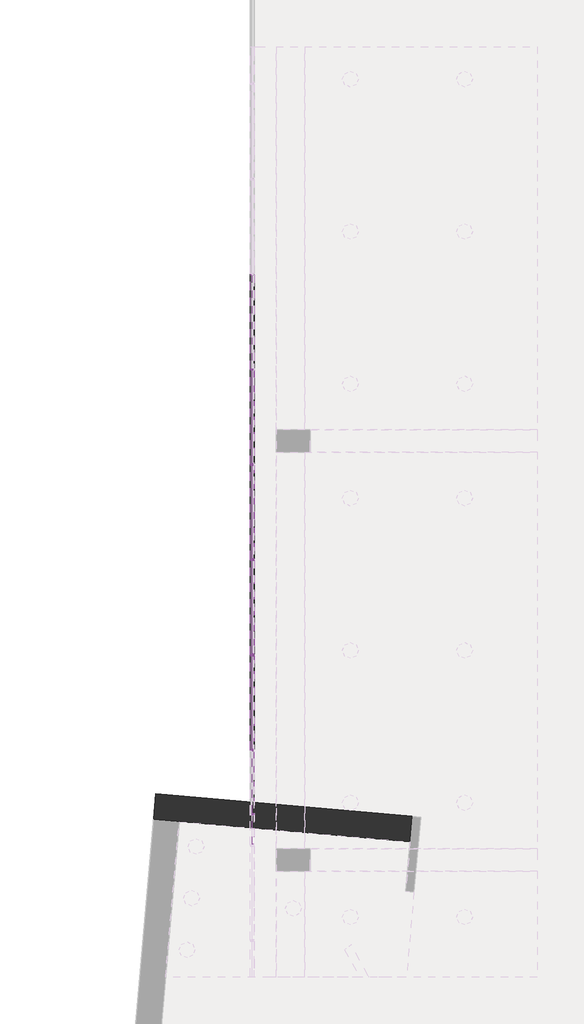
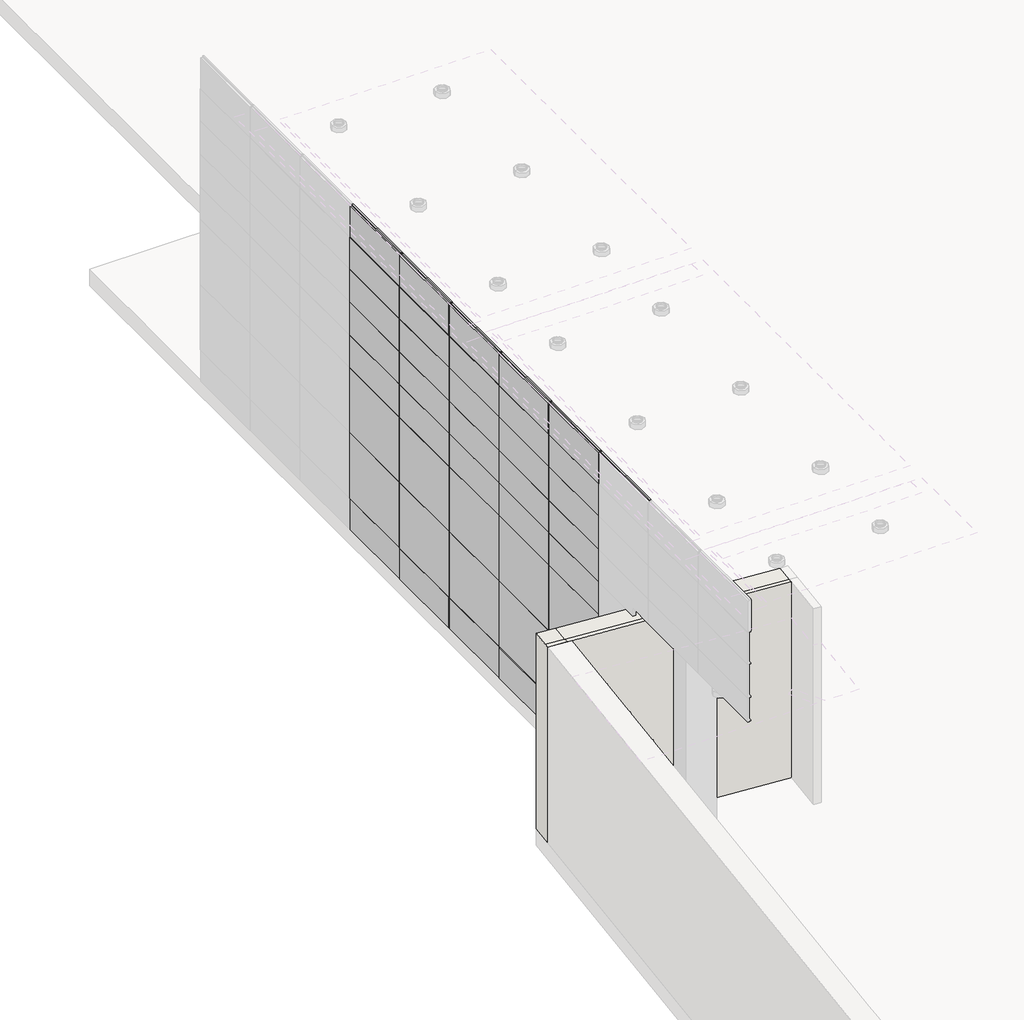
# One storey, part 6 of 30: 90 members, 40 plates, 1 wall.
# Revit data of these elements (continued)
# Project information
#   Project Issue Date = "Issue Date"
#   Project Status = "Project Status"
#   Client Name = "Owner"
#   Project Address = "Enter address here"
#   Project Name = "Project Name"
#   Project Number = "Project Number"
# Grids (mm)
#   "9.6": line (6864.976, -37283.911) -> (5806.021, -17077.846)
#   "G.5": line (37124.427, -17190.111) -> (-12577.847, -19794.897)
#   "H.5": line (37384.644, -22155.347) -> (-12317.63, -24760.133)
#   "J.5": line (37756.193, -29244.918) -> (-11946.082, -31849.704)
#   "K": line (37958.916, -33113.109) -> (-11743.358, -35717.895)
#   "F.5": line (36725.627, -9580.554) -> (10926.266, -10932.641)
#   "E.5": line (36326.827, -1970.997) -> (10527.466, -3323.084)
#   "C.5": line (35928.027, 5638.56) -> (10128.666, 4286.473)
#   "7.2": line (-9673.128, -38150.636) -> (-10732.083, -17944.571)
#   "8.4": line (-1404.076, -37717.274) -> (-2463.031, -17511.208)
#   "10.8": line (15894.983, -36810.669) -> (14836.028, -16604.603)
#   "13": line (34795.221, -35820.149) -> (33736.266, -15614.084)
#   "1": line (-51461.944, -37576.833) -> (-51461.944, 28762.958)
#   "2": line (-45365.944, -37576.833) -> (-45365.944, 28762.958)
#   "3": line (-38050.744, -37576.833) -> (-38050.744, 28762.958)
#   "4": line (-31345.144, -37576.833) -> (-31345.144, 28762.958)
#   "5": line (-24639.544, -37576.833) -> (-24639.544, 28762.958)
#   "6": line (-17933.944, -37576.833) -> (-17933.944, 28762.958)
#   "7": line (-11228.344, -37576.833) -> (-11228.344, 28762.958)
#   "8": line (-4522.744, -37576.833) -> (-4522.744, 28762.958)
#   "9": line (2182.856, -37576.833) -> (2182.856, 28762.958)
#   "10": line (8888.456, -37576.833) -> (8888.456, 28762.958)
#   "11": line (16203.656, -37576.833) -> (16203.656, 28762.958)
#   "12": line (22299.656, -37576.833) -> (22299.656, 28762.958)
#   "A": line (38014.081, 14523.24) -> (-59082, 14523.24)
#   "B": line (38014.081, 10865.64) -> (-59082, 10865.64)
#   "C": line (38014.081, 7512.84) -> (-59082, 7512.84)
#   "D": line (38014.081, 4160.04) -> (-59082, 4160.04)
#   "E": line (38014.081, 807.24) -> (-59082, 807.24)
#   "F": line (38014.081, -5898.36) -> (-59082, -5898.36)
#   "G": line (38014.081, -12603.96) -> (-59082, -12603.96)
#   "H": line (38014.081, -19309.56) -> (-59082, -19309.56)
#   "J": line (38014.081, -25405.56) -> (-59082, -25405.56)
# Type "Rectangular Mullion : 1\" Square"
#   built-in parameter 1007304 = 0.0833333 (stored number, unit not read)
#   built-in parameter 1007301 = 0.0416667 (stored number, unit not read)
#   built-in parameter 1007300 = 0.0416667 (stored number, unit not read)
# Type "Generic - 13+3 1/8\""
#   Assembly Code = "B2010"
#   Layers, outside or top first: 330.2 mm no material (function 1); 79.375 mm no material (function 1)
# Elements 1, 2, 3, 4, 5, 6, 7, 8, 9, 10, 11, 12, 13, 14, 15, 16, 17, 18, 19, 20, 21, 22, 23, 24, 25, 26, 27, 28, 29, 30, 31, 32, 33, 34, 35, 36, 37, 38, 39, 40, 41, 42, 43, 44, 45, 46, 47, 48, 49, 50, 51, 52, 53, 54, 55, 56, 57, 58, 59, 60, 61, 62, 63, 64, 65, 66, 67, 68, 69, 70, 71, 72, 73, 74, 75, 76, 77, 78, 79, 80, 81, 82, 83, 84, 85, 86, 87, 88, 89, 90 (IfcMember, "Rectangular Mullion : 1\" Square")
#   Phase Created = New Construction
#   Materials on its faces: "Metal - Aluminum"
# Elements 91, 92, 93, 94, 95, 96, 97, 98, 99, 100, 101, 102, 103, 104, 105, 106, 107, 108, 109, 110, 111, 112, 113, 114, 115, 116, 117, 118, 119, 120 (IfcPlate, "System Panel : Glazed")
#   Phase Created = New Construction
#   Materials on its faces: "Glass"
# Elements 121, 122, 123, 124, 125, 126, 127, 128, 129, 130 (IfcPlate, "System Panel : Solid")
#   Phase Created = New Construction
#   Materials on its faces: "Default"
# Element 131 (IfcWall, "Generic - 13+3 1/8\"")
#   Top Offset = 0 mm
#   Base Offset = 0 mm
#   wall height = 3657.6 mm
#   Phase Created = New Construction
#   Base Constraint = 1ST. FL.
#   Top Constraint = 2ND FL.
#   Materials on its faces: "Default Wall"
# Materials
#   "Metal - Aluminum": class "Metal", colour RGB 247 247 247, transparency 0
#   "Glass": class "Glass", colour RGB 0 128 192, transparency 0.75
#   "Default": class "Miscellaneous", colour RGB 127 127 127, transparency 0
#   "Default Wall": class "Miscellaneous", colour RGB 128 128 128, transparency 0
# Space at (-50350.74, -30466.395) mm, phase "New Construction", upper level "1ST. FL.", upper offset 3048 mm, lower offset 0 mm
#   Number = "20"
#   Name = "Space"
#   Actual Lighting Load per area = 0
#   Actual Power Load per area = 0
#   Sensible Heat Gain per person = 0
#   Specified Lighting Load = 153.554 (stored number, unit not read)
#   Specified Power Load = 199.62 (stored number, unit not read)
#   Latent Heat Gain per person = 0
#   Total Heat Gain per person = 0
#   Area per Person = 0
#   Number of People = 0.0463862 (stored number, unit not read)
#   Lighting Load Units = 0
#   Power Load Units = 0
#   Return Airflow = 0
#   Occupancy Unit = -1
#   Condition Type = 2
#   Construction Type = none
# Space at (-51280.638, -30385.039) mm, phase "New Construction", upper level "1ST. FL.", upper offset 3048 mm, lower offset 0 mm
#   Number = "21"
#   Name = "Space"
#   Actual Lighting Load per area = 0
#   Actual Power Load per area = 0
#   Sensible Heat Gain per person = 0
#   Specified Lighting Load = 153.554 (stored number, unit not read)
#   Specified Power Load = 199.62 (stored number, unit not read)
#   Latent Heat Gain per person = 0
#   Total Heat Gain per person = 0
#   Area per Person = 0
#   Number of People = 0.0463862 (stored number, unit not read)
#   Lighting Load Units = 0
#   Power Load Units = 0
#   Return Airflow = 0
#   Occupancy Unit = -1
#   Condition Type = 2
#   Construction Type = none
# Space at (-52210.536, -30303.684) mm, phase "New Construction", upper level "1ST. FL.", upper offset 3048 mm, lower offset 0 mm
#   Number = "22"
#   Name = "Space"
#   Actual Lighting Load per area = 0
#   Actual Power Load per area = 0
#   Sensible Heat Gain per person = 0
#   Specified Lighting Load = 153.554 (stored number, unit not read)
#   Specified Power Load = 199.62 (stored number, unit not read)
#   Latent Heat Gain per person = 0
#   Total Heat Gain per person = 0
#   Area per Person = 0
#   Number of People = 0.0463862 (stored number, unit not read)
#   Lighting Load Units = 0
#   Power Load Units = 0
#   Return Airflow = 0
#   Occupancy Unit = -1
#   Condition Type = 2
#   Construction Type = none
# Space at (-52088.521, -24227.572) mm, phase "New Construction", upper level "1ST. FL.", upper offset 3048 mm, lower offset 0 mm
#   Number = "23"
#   Name = "Space"
#   Actual Lighting Load per area = 0
#   Actual Power Load per area = 0
#   Sensible Heat Gain per person = 0
#   Specified Lighting Load = 3477.7 (stored number, unit not read)
#   Specified Power Load = 4521.01 (stored number, unit not read)
#   Latent Heat Gain per person = 0
#   Total Heat Gain per person = 0
#   Area per Person = 0
#   Number of People = 1.05056 (stored number, unit not read)
#   Lighting Load Units = 0
#   Power Load Units = 0
#   Return Airflow = 0
#   Occupancy Unit = -1
#   Condition Type = 2
#   Construction Type = none
# Space at (-51998.779, -31381.93) mm, phase "New Construction", upper level "1ST. FL.", upper offset 3048 mm, lower offset 0 mm
#   Number = "24"
#   Name = "Space"
#   Actual Lighting Load per area = 0
#   Actual Power Load per area = 0
#   Sensible Heat Gain per person = 0
#   Specified Lighting Load = 909.282 (stored number, unit not read)
#   Specified Power Load = 1182.07 (stored number, unit not read)
#   Latent Heat Gain per person = 0
#   Total Heat Gain per person = 0
#   Area per Person = 0
#   Number of People = 0.27468 (stored number, unit not read)
#   Lighting Load Units = 0
#   Power Load Units = 0
#   Return Airflow = 0
#   Occupancy Unit = -1
#   Condition Type = 2
#   Construction Type = none
# Space at (15225.756, -15893.26) mm, phase "New Construction", upper level "1ST. FL.", upper offset 3048 mm, lower offset 0 mm
#   Number = "29"
#   Name = "Space"
#   Actual Lighting Load per area = 0
#   Actual Power Load per area = 0
#   Sensible Heat Gain per person = 0
#   Specified Lighting Load = 62.8642 (stored number, unit not read)
#   Specified Power Load = 81.7235 (stored number, unit not read)
#   Latent Heat Gain per person = 0
#   Total Heat Gain per person = 0
#   Area per Person = 0
#   Number of People = 0.0189903 (stored number, unit not read)
#   Lighting Load Units = 0
#   Power Load Units = 0
#   Return Airflow = 0
#   Occupancy Unit = -1
#   Condition Type = 2
#   Construction Type = none
# Space at (-10682.244, -17819.949) mm, phase "New Construction", upper level "1ST. FL.", upper offset 3048 mm, lower offset 0 mm
#   Number = "30"
#   Name = "Space"
#   Actual Lighting Load per area = 0
#   Actual Power Load per area = 0
#   Sensible Heat Gain per person = 0
#   Specified Lighting Load = 1649.25 (stored number, unit not read)
#   Specified Power Load = 2144.03 (stored number, unit not read)
#   Latent Heat Gain per person = 0
#   Total Heat Gain per person = 0
#   Area per Person = 0
#   Number of People = 0.498213 (stored number, unit not read)
#   Lighting Load Units = 0
#   Power Load Units = 0
#   Return Airflow = 0
#   Occupancy Unit = -1
#   Condition Type = 2
#   Construction Type = none
# Space at (-39.644, -17389.234) mm, phase "New Construction", upper level "1ST. FL.", upper offset 3048 mm, lower offset 0 mm
#   Number = "31"
#   Name = "Space"
#   Actual Lighting Load per area = 0
#   Actual Power Load per area = 0
#   Sensible Heat Gain per person = 0
#   Specified Lighting Load = 525.995 (stored number, unit not read)
#   Specified Power Load = 683.794 (stored number, unit not read)
#   Latent Heat Gain per person = 0
#   Total Heat Gain per person = 0
#   Area per Person = 0
#   Number of People = 0.158895 (stored number, unit not read)
#   Lighting Load Units = 0
#   Power Load Units = 0
#   Return Airflow = 0
#   Occupancy Unit = -1
#   Condition Type = 2
#   Construction Type = none
# Space at (2182.856, 13850.14) mm, phase "New Construction", upper level "1ST. FL.", upper offset 3048 mm, lower offset 0 mm
#   Number = "36"
#   Name = "Space"
#   Actual Lighting Load per area = 0
#   Actual Power Load per area = 0
#   Sensible Heat Gain per person = 0
#   Specified Lighting Load = 134.399 (stored number, unit not read)
#   Specified Power Load = 174.719 (stored number, unit not read)
#   Latent Heat Gain per person = 0
#   Total Heat Gain per person = 0
#   Area per Person = 0
#   Number of People = 0.0405999 (stored number, unit not read)
#   Lighting Load Units = 0
#   Power Load Units = 0
#   Return Airflow = 0
#   Occupancy Unit = -1
#   Condition Type = 2
#   Construction Type = none
# Space at (-44388.044, -15893.26) mm, phase "New Construction", upper level "1ST. FL.", upper offset 3048 mm, lower offset 0 mm
#   Number = "37"
#   Name = "Space"
#   Actual Lighting Load per area = 0
#   Actual Power Load per area = 0
#   Sensible Heat Gain per person = 0
#   Specified Lighting Load = 62.8642 (stored number, unit not read)
#   Specified Power Load = 81.7235 (stored number, unit not read)
#   Latent Heat Gain per person = 0
#   Total Heat Gain per person = 0
#   Area per Person = 0
#   Number of People = 0.0189903 (stored number, unit not read)
#   Lighting Load Units = 0
#   Power Load Units = 0
#   Return Airflow = 0
#   Occupancy Unit = -1
#   Condition Type = 2
#   Construction Type = none
# Space at (-31345.144, 13850.14) mm, phase "New Construction", upper level "1ST. FL.", upper offset 3048 mm, lower offset 0 mm
#   Number = "40"
#   Name = "Space"
#   Actual Lighting Load per area = 0
#   Actual Power Load per area = 0
#   Sensible Heat Gain per person = 0
#   Specified Lighting Load = 134.399 (stored number, unit not read)
#   Specified Power Load = 174.719 (stored number, unit not read)
#   Latent Heat Gain per person = 0
#   Total Heat Gain per person = 0
#   Area per Person = 0
#   Number of People = 0.0405999 (stored number, unit not read)
#   Lighting Load Units = 0
#   Power Load Units = 0
#   Return Airflow = 0
#   Occupancy Unit = -1
#   Condition Type = 2
#   Construction Type = none
# Space at (-14581.144, -2215.36) mm, phase "New Construction", upper level "1ST. FL.", upper offset 3048 mm, lower offset 0 mm
#   Number = "41"
#   Name = "Space"
#   Actual Lighting Load per area = 0
#   Actual Power Load per area = 0
#   Sensible Heat Gain per person = 0
#   Specified Lighting Load = 213384.3 (stored number, unit not read)
#   Specified Power Load = 277399.6 (stored number, unit not read)
#   Latent Heat Gain per person = 0
#   Total Heat Gain per person = 0
#   Area per Person = 0
#   Number of People = 64.46 (stored number, unit not read)
#   Lighting Load Units = 0
#   Power Load Units = 0
#   Return Airflow = 0
#   Occupancy Unit = -1
#   Condition Type = 2
#   Construction Type = none
# Space at (-22969.494, 18968.24) mm, phase "New Construction", upper level "1ST. FL.", upper offset 3048 mm, lower offset 0 mm
#   Number = "44"
#   Name = "Space"
#   Actual Lighting Load per area = 0
#   Actual Power Load per area = 0
#   Sensible Heat Gain per person = 0
#   Specified Lighting Load = 1066.26 (stored number, unit not read)
#   Specified Power Load = 1386.14 (stored number, unit not read)
#   Latent Heat Gain per person = 0
#   Total Heat Gain per person = 0
#   Area per Person = 0
#   Number of People = 0.322101 (stored number, unit not read)
#   Lighting Load Units = 0
#   Power Load Units = 0
#   Return Airflow = 0
#   Occupancy Unit = -1
#   Condition Type = 2
#   Construction Type = none
# Space at (-19896.094, 18968.24) mm, phase "New Construction", upper level "1ST. FL.", upper offset 3048 mm, lower offset 0 mm
#   Number = "45"
#   Name = "Space"
#   Actual Lighting Load per area = 0
#   Actual Power Load per area = 0
#   Sensible Heat Gain per person = 0
#   Specified Lighting Load = 560.359 (stored number, unit not read)
#   Specified Power Load = 728.466 (stored number, unit not read)
#   Latent Heat Gain per person = 0
#   Total Heat Gain per person = 0
#   Area per Person = 0
#   Number of People = 0.169275 (stored number, unit not read)
#   Lighting Load Units = 0
#   Power Load Units = 0
#   Return Airflow = 0
#   Occupancy Unit = -1
#   Condition Type = 2
#   Construction Type = none
# Space at (-18559.419, 18968.24) mm, phase "New Construction", upper level "1ST. FL.", upper offset 3048 mm, lower offset 0 mm
#   Number = "46"
#   Name = "Space"
#   Actual Lighting Load per area = 0
#   Actual Power Load per area = 0
#   Sensible Heat Gain per person = 0
#   Specified Lighting Load = 99.2485 (stored number, unit not read)
#   Specified Power Load = 129.023 (stored number, unit not read)
#   Latent Heat Gain per person = 0
#   Total Heat Gain per person = 0
#   Area per Person = 0
#   Number of People = 0.0299814 (stored number, unit not read)
#   Lighting Load Units = 0
#   Power Load Units = 0
#   Return Airflow = 0
#   Occupancy Unit = -1
#   Condition Type = 2
#   Construction Type = none
# Space at (-33885.144, 21730.49) mm, phase "New Construction", upper level "1ST. FL.", upper offset 3048 mm, lower offset 0 mm
#   Number = "47"
#   Name = "Space"
#   Actual Lighting Load per area = 0
#   Actual Power Load per area = 0
#   Sensible Heat Gain per person = 0
#   Specified Lighting Load = 18748.3 (stored number, unit not read)
#   Specified Power Load = 24372.8 (stored number, unit not read)
#   Latent Heat Gain per person = 0
#   Total Heat Gain per person = 0
#   Area per Person = 0
#   Number of People = 5.66358 (stored number, unit not read)
#   Lighting Load Units = 0
#   Power Load Units = 0
#   Return Airflow = 0
#   Occupancy Unit = -1
#   Condition Type = 2
#   Construction Type = none
# Space at (-34520.144, 24245.09) mm, phase "New Construction", upper level "1ST. FL.", upper offset 3048 mm, lower offset 0 mm
#   Number = "48"
#   Name = "Space"
#   Actual Lighting Load per area = 0
#   Actual Power Load per area = 0
#   Sensible Heat Gain per person = 0
#   Specified Lighting Load = 746.746 (stored number, unit not read)
#   Specified Power Load = 970.77 (stored number, unit not read)
#   Latent Heat Gain per person = 0
#   Total Heat Gain per person = 0
#   Area per Person = 0
#   Number of People = 0.22558 (stored number, unit not read)
#   Lighting Load Units = 0
#   Power Load Units = 0
#   Return Airflow = 0
#   Occupancy Unit = -1
#   Condition Type = 2
#   Construction Type = none
# Space at (-32361.144, 24245.09) mm, phase "New Construction", upper level "1ST. FL.", upper offset 3048 mm, lower offset 0 mm
#   Number = "49"
#   Name = "Space"
#   Actual Lighting Load per area = 0
#   Actual Power Load per area = 0
#   Sensible Heat Gain per person = 0
#   Specified Lighting Load = 547.614 (stored number, unit not read)
#   Specified Power Load = 711.898 (stored number, unit not read)
#   Latent Heat Gain per person = 0
#   Total Heat Gain per person = 0
#   Area per Person = 0
#   Number of People = 0.165425 (stored number, unit not read)
#   Lighting Load Units = 0
#   Power Load Units = 0
#   Return Airflow = 0
#   Occupancy Unit = -1
#   Condition Type = 2
#   Construction Type = none
# Space at (-29490.944, 24245.09) mm, phase "New Construction", upper level "1ST. FL.", upper offset 3048 mm, lower offset 0 mm
#   Number = "50"
#   Name = "Space"
#   Actual Lighting Load per area = 0
#   Actual Power Load per area = 0
#   Sensible Heat Gain per person = 0
#   Specified Lighting Load = 1211.39 (stored number, unit not read)
#   Specified Power Load = 1574.8 (stored number, unit not read)
#   Latent Heat Gain per person = 0
#   Total Heat Gain per person = 0
#   Area per Person = 0
#   Number of People = 0.365941 (stored number, unit not read)
#   Lighting Load Units = 0
#   Power Load Units = 0
#   Return Airflow = 0
#   Occupancy Unit = -1
#   Condition Type = 2
#   Construction Type = none
# Space at (-20670.794, 24245.09) mm, phase "New Construction", upper level "1ST. FL.", upper offset 3048 mm, lower offset 0 mm
#   Number = "51"
#   Name = "Space"
#   Actual Lighting Load per area = 0
#   Actual Power Load per area = 0
#   Sensible Heat Gain per person = 0
#   Specified Lighting Load = 1510.09 (stored number, unit not read)
#   Specified Power Load = 1963.11 (stored number, unit not read)
#   Latent Heat Gain per person = 0
#   Total Heat Gain per person = 0
#   Area per Person = 0
#   Number of People = 0.456173 (stored number, unit not read)
#   Lighting Load Units = 0
#   Power Load Units = 0
#   Return Airflow = 0
#   Occupancy Unit = -1
#   Condition Type = 2
#   Construction Type = none
# Space at (15876.631, 9189.24) mm, phase "New Construction", upper level "1ST. FL.", upper offset 3048 mm, lower offset 0 mm
#   Number = "53"
#   Name = "Space"
#   Actual Lighting Load per area = 0
#   Actual Power Load per area = 0
#   Sensible Heat Gain per person = 0
#   Specified Lighting Load = 68.1434 (stored number, unit not read)
#   Specified Power Load = 88.5864 (stored number, unit not read)
#   Latent Heat Gain per person = 0
#   Total Heat Gain per person = 0
#   Area per Person = 0
#   Number of People = 0.020585 (stored number, unit not read)
#   Lighting Load Units = 0
#   Power Load Units = 0
#   Return Airflow = 0
#   Occupancy Unit = -1
#   Condition Type = 2
#   Construction Type = none
# Space at (15876.631, 6550.815) mm, phase "New Construction", upper level "1ST. FL.", upper offset 3048 mm, lower offset 0 mm
#   Number = "54"
#   Name = "Space"
#   Actual Lighting Load per area = 0
#   Actual Power Load per area = 0
#   Sensible Heat Gain per person = 0
#   Specified Lighting Load = 33.455 (stored number, unit not read)
#   Specified Power Load = 43.4915 (stored number, unit not read)
#   Latent Heat Gain per person = 0
#   Total Heat Gain per person = 0
#   Area per Person = 0
#   Number of People = 0.0101062 (stored number, unit not read)
#   Lighting Load Units = 0
#   Power Load Units = 0
#   Return Airflow = 0
#   Occupancy Unit = -1
#   Condition Type = 2
#   Construction Type = none
# Space at (-5629.232, 19134.928) mm, phase "New Construction", upper level "1ST. FL.", upper offset 3048 mm, lower offset 0 mm
#   Number = "55"
#   Name = "Space"
#   Actual Lighting Load per area = 0
#   Actual Power Load per area = 0
#   Sensible Heat Gain per person = 0
#   Specified Lighting Load = 837.567 (stored number, unit not read)
#   Specified Power Load = 1088.84 (stored number, unit not read)
#   Latent Heat Gain per person = 0
#   Total Heat Gain per person = 0
#   Area per Person = 0
#   Number of People = 0.253016 (stored number, unit not read)
#   Lighting Load Units = 0
#   Power Load Units = 0
#   Return Airflow = 0
#   Occupancy Unit = -1
#   Condition Type = 2
#   Construction Type = none
# Space at (5749.822, 21730.49) mm, phase "New Construction", upper level "1ST. FL.", upper offset 3048 mm, lower offset 0 mm
#   Number = "56"
#   Name = "Space"
#   Actual Lighting Load per area = 0
#   Actual Power Load per area = 0
#   Sensible Heat Gain per person = 0
#   Specified Lighting Load = 21109.8 (stored number, unit not read)
#   Specified Power Load = 27442.8 (stored number, unit not read)
#   Latent Heat Gain per person = 0
#   Total Heat Gain per person = 0
#   Area per Person = 0
#   Number of People = 6.37694 (stored number, unit not read)
#   Lighting Load Units = 0
#   Power Load Units = 0
#   Return Airflow = 0
#   Occupancy Unit = -1
#   Condition Type = 2
#   Construction Type = none
# Space at (-8974.094, 22176.578) mm, phase "New Construction", upper level "1ST. FL.", upper offset 3048 mm, lower offset 0 mm
#   Number = "57"
#   Name = "Space"
#   Actual Lighting Load per area = 0
#   Actual Power Load per area = 0
#   Sensible Heat Gain per person = 0
#   Specified Lighting Load = 2957.38 (stored number, unit not read)
#   Specified Power Load = 3844.6 (stored number, unit not read)
#   Latent Heat Gain per person = 0
#   Total Heat Gain per person = 0
#   Area per Person = 0
#   Number of People = 0.893379 (stored number, unit not read)
#   Lighting Load Units = 0
#   Power Load Units = 0
#   Return Airflow = 0
#   Occupancy Unit = -1
#   Condition Type = 2
#   Construction Type = none
# Space at (-44969.069, -12603.96) mm, phase "New Construction", upper level "1ST. FL.", upper offset 3048 mm, lower offset 0 mm
#   Number = "58"
#   Name = "Space"
#   Actual Lighting Load per area = 0
#   Actual Power Load per area = 0
#   Sensible Heat Gain per person = 0
#   Specified Lighting Load = 3.50388 (stored number, unit not read)
#   Specified Power Load = 4.55504 (stored number, unit not read)
#   Latent Heat Gain per person = 0
#   Total Heat Gain per person = 0
#   Area per Person = 0
#   Number of People = 0.00105847 (stored number, unit not read)
#   Lighting Load Units = 0
#   Power Load Units = 0
#   Return Airflow = 0
#   Occupancy Unit = -1
#   Condition Type = 2
#   Construction Type = none
# Space at (-42459.607, -28070.561) mm, phase "New Construction", upper level "1ST. FL.", upper offset 3048 mm, lower offset 0 mm
#   Number = "59"
#   Name = "Space"
#   Actual Lighting Load per area = 0
#   Actual Power Load per area = 0
#   Sensible Heat Gain per person = 0
#   Specified Lighting Load = 2731.52 (stored number, unit not read)
#   Specified Power Load = 3550.97 (stored number, unit not read)
#   Latent Heat Gain per person = 0
#   Total Heat Gain per person = 0
#   Area per Person = 0
#   Number of People = 0.825148 (stored number, unit not read)
#   Lighting Load Units = 0
#   Power Load Units = 0
#   Return Airflow = 0
#   Occupancy Unit = -1
#   Condition Type = 2
#   Construction Type = none
# Space at (15806.781, 807.24) mm, phase "New Construction", upper level "1ST. FL.", upper offset 3048 mm, lower offset 0 mm
#   Number = "62"
#   Name = "Space"
#   Actual Lighting Load per area = 0
#   Actual Power Load per area = 0
#   Sensible Heat Gain per person = 0
#   Specified Lighting Load = 3.50388 (stored number, unit not read)
#   Specified Power Load = 4.55504 (stored number, unit not read)
#   Latent Heat Gain per person = 0
#   Total Heat Gain per person = 0
#   Area per Person = 0
#   Number of People = 0.00105847 (stored number, unit not read)
#   Lighting Load Units = 0
#   Power Load Units = 0
#   Return Airflow = 0
#   Occupancy Unit = -1
#   Condition Type = 2
#   Construction Type = none
# Space at (-44969.069, -5898.36) mm, phase "New Construction", upper level "1ST. FL.", upper offset 3048 mm, lower offset 0 mm
#   Number = "63"
#   Name = "Space"
#   Actual Lighting Load per area = 0
#   Actual Power Load per area = 0
#   Sensible Heat Gain per person = 0
#   Specified Lighting Load = 3.50388 (stored number, unit not read)
#   Specified Power Load = 4.55504 (stored number, unit not read)
#   Latent Heat Gain per person = 0
#   Total Heat Gain per person = 0
#   Area per Person = 0
#   Number of People = 0.00105847 (stored number, unit not read)
#   Lighting Load Units = 0
#   Power Load Units = 0
#   Return Airflow = 0
#   Occupancy Unit = -1
#   Condition Type = 2
#   Construction Type = none
# Space at (-44969.069, 807.24) mm, phase "New Construction", upper level "1ST. FL.", upper offset 3048 mm, lower offset 0 mm
#   Number = "64"
#   Name = "Space"
#   Actual Lighting Load per area = 0
#   Actual Power Load per area = 0
#   Sensible Heat Gain per person = 0
#   Specified Lighting Load = 3.50388 (stored number, unit not read)
#   Specified Power Load = 4.55504 (stored number, unit not read)
#   Latent Heat Gain per person = 0
#   Total Heat Gain per person = 0
#   Area per Person = 0
#   Number of People = 0.00105847 (stored number, unit not read)
#   Lighting Load Units = 0
#   Power Load Units = 0
#   Return Airflow = 0
#   Occupancy Unit = -1
#   Condition Type = 2
#   Construction Type = none
# Space at (-15300.665, 15209.103) mm, phase "New Construction", upper level "1ST. FL.", upper offset 3048 mm, lower offset 0 mm
#   Number = "65"
#   Name = "Space"
#   Actual Lighting Load per area = 0
#   Actual Power Load per area = 0
#   Sensible Heat Gain per person = 0
#   Specified Lighting Load = 29471.5 (stored number, unit not read)
#   Specified Power Load = 38312.9 (stored number, unit not read)
#   Latent Heat Gain per person = 0
#   Total Heat Gain per person = 0
#   Area per Person = 0
#   Number of People = 8.90286 (stored number, unit not read)
#   Lighting Load Units = 0
#   Power Load Units = 0
#   Return Airflow = 0
#   Occupancy Unit = -1
#   Condition Type = 2
#   Construction Type = none
# Space at (15806.781, 10865.64) mm, phase "New Construction", upper level "1ST. FL.", upper offset 3048 mm, lower offset 0 mm
#   Number = "66"
#   Name = "Space"
#   Actual Lighting Load per area = 0
#   Actual Power Load per area = 0
#   Sensible Heat Gain per person = 0
#   Specified Lighting Load = 3.50388 (stored number, unit not read)
#   Specified Power Load = 4.55504 (stored number, unit not read)
#   Latent Heat Gain per person = 0
#   Total Heat Gain per person = 0
#   Area per Person = 0
#   Number of People = 0.00105847 (stored number, unit not read)
#   Lighting Load Units = 0
#   Power Load Units = 0
#   Return Airflow = 0
#   Occupancy Unit = -1
#   Condition Type = 2
#   Construction Type = none
# Space at (15806.781, 7512.84) mm, phase "New Construction", upper level "1ST. FL.", upper offset 3048 mm, lower offset 0 mm
#   Number = "67"
#   Name = "Space"
#   Actual Lighting Load per area = 0
#   Actual Power Load per area = 0
#   Sensible Heat Gain per person = 0
#   Specified Lighting Load = 3.50388 (stored number, unit not read)
#   Specified Power Load = 4.55504 (stored number, unit not read)
#   Latent Heat Gain per person = 0
#   Total Heat Gain per person = 0
#   Area per Person = 0
#   Number of People = 0.00105847 (stored number, unit not read)
#   Lighting Load Units = 0
#   Power Load Units = 0
#   Return Airflow = 0
#   Occupancy Unit = -1
#   Condition Type = 2
#   Construction Type = none
# Space at (-44969.069, 7512.84) mm, phase "New Construction", upper level "1ST. FL.", upper offset 3048 mm, lower offset 0 mm
#   Number = "68"
#   Name = "Space"
#   Actual Lighting Load per area = 0
#   Actual Power Load per area = 0
#   Sensible Heat Gain per person = 0
#   Specified Lighting Load = 3.50388 (stored number, unit not read)
#   Specified Power Load = 4.55504 (stored number, unit not read)
#   Latent Heat Gain per person = 0
#   Total Heat Gain per person = 0
#   Area per Person = 0
#   Number of People = 0.00105847 (stored number, unit not read)
#   Lighting Load Units = 0
#   Power Load Units = 0
#   Return Airflow = 0
#   Occupancy Unit = -1
#   Condition Type = 2
#   Construction Type = none
# Space at (-44969.069, 4160.04) mm, phase "New Construction", upper level "1ST. FL.", upper offset 3048 mm, lower offset 0 mm
#   Number = "69"
#   Name = "Space"
#   Actual Lighting Load per area = 0
#   Actual Power Load per area = 0
#   Sensible Heat Gain per person = 0
#   Specified Lighting Load = 3.50388 (stored number, unit not read)
#   Specified Power Load = 4.55504 (stored number, unit not read)
#   Latent Heat Gain per person = 0
#   Total Heat Gain per person = 0
#   Area per Person = 0
#   Number of People = 0.00105847 (stored number, unit not read)
#   Lighting Load Units = 0
#   Power Load Units = 0
#   Return Airflow = 0
#   Occupancy Unit = -1
#   Condition Type = 2
#   Construction Type = none
# Space at (-2305.302, -27806.676) mm, phase "New Construction", upper level "1ST. FL.", upper offset 3048 mm, lower offset 0 mm
#   Number = "70"
#   Name = "Space"
#   Actual Lighting Load per area = 0
#   Actual Power Load per area = 0
#   Sensible Heat Gain per person = 0
#   Specified Lighting Load = 979.316 (stored number, unit not read)
#   Specified Power Load = 1273.11 (stored number, unit not read)
#   Latent Heat Gain per person = 0
#   Total Heat Gain per person = 0
#   Area per Person = 0
#   Number of People = 0.295836 (stored number, unit not read)
#   Lighting Load Units = 0
#   Power Load Units = 0
#   Return Airflow = 0
#   Occupancy Unit = -1
#   Condition Type = 2
#   Construction Type = none
# Space at (427.548, -27351.224) mm, phase "New Construction", upper level "1ST. FL.", upper offset 3048 mm, lower offset 0 mm
#   Number = "71"
#   Name = "Space"
#   Actual Lighting Load per area = 0
#   Actual Power Load per area = 0
#   Sensible Heat Gain per person = 0
#   Specified Lighting Load = 1259.38 (stored number, unit not read)
#   Specified Power Load = 1637.19 (stored number, unit not read)
#   Latent Heat Gain per person = 0
#   Total Heat Gain per person = 0
#   Area per Person = 0
#   Number of People = 0.380438 (stored number, unit not read)
#   Lighting Load Units = 0
#   Power Load Units = 0
#   Return Airflow = 0
#   Occupancy Unit = -1
#   Condition Type = 2
#   Construction Type = none
# Space at (287.151, -24805.774) mm, phase "New Construction", upper level "1ST. FL.", upper offset 3048 mm, lower offset 0 mm
#   Number = "72"
#   Name = "Space"
#   Actual Lighting Load per area = 0
#   Actual Power Load per area = 0
#   Sensible Heat Gain per person = 0
#   Specified Lighting Load = 285.033 (stored number, unit not read)
#   Specified Power Load = 370.542 (stored number, unit not read)
#   Latent Heat Gain per person = 0
#   Total Heat Gain per person = 0
#   Area per Person = 0
#   Number of People = 0.0861038 (stored number, unit not read)
#   Lighting Load Units = 0
#   Power Load Units = 0
#   Return Airflow = 0
#   Occupancy Unit = -1
#   Condition Type = 2
#   Construction Type = none
# Space at (-4916.12, -27061.973) mm, phase "New Construction", upper level "1ST. FL.", upper offset 3048 mm, lower offset 0 mm
#   Number = "73"
#   Name = "Space"
#   Actual Lighting Load per area = 0
#   Actual Power Load per area = 0
#   Sensible Heat Gain per person = 0
#   Specified Lighting Load = 1376.65 (stored number, unit not read)
#   Specified Power Load = 1789.64 (stored number, unit not read)
#   Latent Heat Gain per person = 0
#   Total Heat Gain per person = 0
#   Area per Person = 0
#   Number of People = 0.415864 (stored number, unit not read)
#   Lighting Load Units = 0
#   Power Load Units = 0
#   Return Airflow = 0
#   Occupancy Unit = -1
#   Condition Type = 2
#   Construction Type = none
# Space at (-6193.624, -24385.796) mm, phase "New Construction", upper level "1ST. FL.", upper offset 3048 mm, lower offset 0 mm
#   Number = "74"
#   Name = "Space"
#   Actual Lighting Load per area = 0
#   Actual Power Load per area = 0
#   Sensible Heat Gain per person = 0
#   Specified Lighting Load = 3.99747 (stored number, unit not read)
#   Specified Power Load = 5.19671 (stored number, unit not read)
#   Latent Heat Gain per person = 0
#   Total Heat Gain per person = 0
#   Area per Person = 0
#   Number of People = 0.00120757 (stored number, unit not read)
#   Lighting Load Units = 0
#   Power Load Units = 0
#   Return Airflow = 0
#   Occupancy Unit = -1
#   Condition Type = 2
#   Construction Type = none
# Space at (-4171.546, -33504.071) mm, phase "New Construction", upper level "1ST. FL.", upper offset 3048 mm, lower offset 0 mm
#   Number = "75"
#   Name = "Space"
#   Actual Lighting Load per area = 0
#   Actual Power Load per area = 0
#   Sensible Heat Gain per person = 0
#   Specified Lighting Load = 1778.74 (stored number, unit not read)
#   Specified Power Load = 2312.36 (stored number, unit not read)
#   Latent Heat Gain per person = 0
#   Total Heat Gain per person = 0
#   Area per Person = 0
#   Number of People = 0.537328 (stored number, unit not read)
#   Lighting Load Units = 0
#   Power Load Units = 0
#   Return Airflow = 0
#   Occupancy Unit = -1
#   Condition Type = 2
#   Construction Type = none
# Space at (3097.933, -26775.812) mm, phase "New Construction", upper level "1ST. FL.", upper offset 3048 mm, lower offset 0 mm
#   Number = "76"
#   Name = "Space"
#   Actual Lighting Load per area = 0
#   Actual Power Load per area = 0
#   Sensible Heat Gain per person = 0
#   Specified Lighting Load = 1438.51 (stored number, unit not read)
#   Specified Power Load = 1870.07 (stored number, unit not read)
#   Latent Heat Gain per person = 0
#   Total Heat Gain per person = 0
#   Area per Person = 0
#   Number of People = 0.434552 (stored number, unit not read)
#   Lighting Load Units = 0
#   Power Load Units = 0
#   Return Airflow = 0
#   Occupancy Unit = -1
#   Condition Type = 2
#   Construction Type = none
# Space at (15459.645, -28932.095) mm, phase "New Construction", upper level "1ST. FL.", upper offset 3048 mm, lower offset 0 mm
#   Number = "77"
#   Name = "Space"
#   Actual Lighting Load per area = 0
#   Actual Power Load per area = 0
#   Sensible Heat Gain per person = 0
#   Specified Lighting Load = 102.724 (stored number, unit not read)
#   Specified Power Load = 133.541 (stored number, unit not read)
#   Latent Heat Gain per person = 0
#   Total Heat Gain per person = 0
#   Area per Person = 0
#   Number of People = 0.0310313 (stored number, unit not read)
#   Lighting Load Units = 0
#   Power Load Units = 0
#   Return Airflow = 0
#   Occupancy Unit = -1
#   Condition Type = 2
#   Construction Type = none
# Space at (14240.113, -29014.839) mm, phase "New Construction", upper level "1ST. FL.", upper offset 3048 mm, lower offset 0 mm
#   Number = "78"
#   Name = "Space"
#   Actual Lighting Load per area = 0
#   Actual Power Load per area = 0
#   Sensible Heat Gain per person = 0
#   Specified Lighting Load = 533.711 (stored number, unit not read)
#   Specified Power Load = 693.824 (stored number, unit not read)
#   Latent Heat Gain per person = 0
#   Total Heat Gain per person = 0
#   Area per Person = 0
#   Number of People = 0.161225 (stored number, unit not read)
#   Lighting Load Units = 0
#   Power Load Units = 0
#   Return Airflow = 0
#   Occupancy Unit = -1
#   Condition Type = 2
#   Construction Type = none
# Space at (12037.866, -27791.919) mm, phase "New Construction", upper level "1ST. FL.", upper offset 3048 mm, lower offset 0 mm
#   Number = "79"
#   Name = "Space"
#   Actual Lighting Load per area = 0
#   Actual Power Load per area = 0
#   Sensible Heat Gain per person = 0
#   Specified Lighting Load = 40.5614 (stored number, unit not read)
#   Specified Power Load = 52.7299 (stored number, unit not read)
#   Latent Heat Gain per person = 0
#   Total Heat Gain per person = 0
#   Area per Person = 0
#   Number of People = 0.012253 (stored number, unit not read)
#   Lighting Load Units = 0
#   Power Load Units = 0
#   Return Airflow = 0
#   Occupancy Unit = -1
#   Condition Type = 2
#   Construction Type = none
# Space at (1956.988, -29737.289) mm, phase "New Construction", upper level "1ST. FL.", upper offset 3048 mm, lower offset 0 mm
#   Number = "80"
#   Name = "Space"
#   Actual Lighting Load per area = 0
#   Actual Power Load per area = 0
#   Sensible Heat Gain per person = 0
#   Specified Lighting Load = 9441.92 (stored number, unit not read)
#   Specified Power Load = 12274.5 (stored number, unit not read)
#   Latent Heat Gain per person = 0
#   Total Heat Gain per person = 0
#   Area per Person = 0
#   Number of People = 2.85225 (stored number, unit not read)
#   Lighting Load Units = 0
#   Power Load Units = 0
#   Return Airflow = 0
#   Occupancy Unit = -1
#   Condition Type = 2
#   Construction Type = none
# Space at (21735.466, 4888.703) mm, phase "New Construction", upper level "1ST. FL.", upper offset 3048 mm, lower offset 0 mm
#   Number = "81"
#   Name = "Space"
#   Actual Lighting Load per area = 0
#   Actual Power Load per area = 0
#   Sensible Heat Gain per person = 0
#   Specified Lighting Load = 193.227 (stored number, unit not read)
#   Specified Power Load = 251.196 (stored number, unit not read)
#   Latent Heat Gain per person = 0
#   Total Heat Gain per person = 0
#   Area per Person = 0
#   Number of People = 0.0583709 (stored number, unit not read)
#   Lighting Load Units = 0
#   Power Load Units = 0
#   Return Airflow = 0
#   Occupancy Unit = -1
#   Condition Type = 2
#   Construction Type = none
# Space at (22320.008, -16889.371) mm, phase "New Construction", upper level "1ST. FL.", upper offset 3048 mm, lower offset 0 mm
#   Number = "82"
#   Name = "Space"
#   Actual Lighting Load per area = 0
#   Actual Power Load per area = 0
#   Sensible Heat Gain per person = 0
#   Specified Lighting Load = 5.21708 (stored number, unit not read)
#   Specified Power Load = 6.78221 (stored number, unit not read)
#   Latent Heat Gain per person = 0
#   Total Heat Gain per person = 0
#   Area per Person = 0
#   Number of People = 0.001576 (stored number, unit not read)
#   Lighting Load Units = 0
#   Power Load Units = 0
#   Return Airflow = 0
#   Occupancy Unit = -1
#   Condition Type = 2
#   Construction Type = none
# Space at (27014.531, 10827.54) mm, phase "New Construction", upper level "1ST. FL.", upper offset 3048 mm, lower offset 0 mm
#   Number = "83"
#   Name = "Space"
#   Actual Lighting Load per area = 0
#   Actual Power Load per area = 0
#   Sensible Heat Gain per person = 0
#   Specified Lighting Load = 153.554 (stored number, unit not read)
#   Specified Power Load = 199.62 (stored number, unit not read)
#   Latent Heat Gain per person = 0
#   Total Heat Gain per person = 0
#   Area per Person = 0
#   Number of People = 0.0463862 (stored number, unit not read)
#   Lighting Load Units = 0
#   Power Load Units = 0
#   Return Airflow = 0
#   Occupancy Unit = -1
#   Condition Type = 2
#   Construction Type = none
# Space at (27947.981, 10827.54) mm, phase "New Construction", upper level "1ST. FL.", upper offset 3048 mm, lower offset 0 mm
#   Number = "84"
#   Name = "Space"
#   Actual Lighting Load per area = 0
#   Actual Power Load per area = 0
#   Sensible Heat Gain per person = 0
#   Specified Lighting Load = 153.554 (stored number, unit not read)
#   Specified Power Load = 199.62 (stored number, unit not read)
#   Latent Heat Gain per person = 0
#   Total Heat Gain per person = 0
#   Area per Person = 0
#   Number of People = 0.0463862 (stored number, unit not read)
#   Lighting Load Units = 0
#   Power Load Units = 0
#   Return Airflow = 0
#   Occupancy Unit = -1
#   Condition Type = 2
#   Construction Type = none
# Space at (28881.431, 10827.54) mm, phase "New Construction", upper level "1ST. FL.", upper offset 3048 mm, lower offset 0 mm
#   Number = "85"
#   Name = "Space"
#   Actual Lighting Load per area = 0
#   Actual Power Load per area = 0
#   Sensible Heat Gain per person = 0
#   Specified Lighting Load = 153.554 (stored number, unit not read)
#   Specified Power Load = 199.62 (stored number, unit not read)
#   Latent Heat Gain per person = 0
#   Total Heat Gain per person = 0
#   Area per Person = 0
#   Number of People = 0.0463862 (stored number, unit not read)
#   Lighting Load Units = 0
#   Power Load Units = 0
#   Return Airflow = 0
#   Occupancy Unit = -1
#   Condition Type = 2
#   Construction Type = none
# Space at (30748.331, 10827.54) mm, phase "New Construction", upper level "1ST. FL.", upper offset 3048 mm, lower offset 0 mm
#   Number = "87"
#   Name = "Space"
#   Actual Lighting Load per area = 0
#   Actual Power Load per area = 0
#   Sensible Heat Gain per person = 0
#   Specified Lighting Load = 153.554 (stored number, unit not read)
#   Specified Power Load = 199.62 (stored number, unit not read)
#   Latent Heat Gain per person = 0
#   Total Heat Gain per person = 0
#   Area per Person = 0
#   Number of People = 0.0463862 (stored number, unit not read)
#   Lighting Load Units = 0
#   Power Load Units = 0
#   Return Airflow = 0
#   Occupancy Unit = -1
#   Condition Type = 2
#   Construction Type = none
# Space at (29649.178, 5573.682) mm, phase "New Construction", upper level "1ST. FL.", upper offset 3048 mm, lower offset 0 mm
#   Number = "88"
#   Name = "Space"
#   Actual Lighting Load per area = 0
#   Actual Power Load per area = 0
#   Sensible Heat Gain per person = 0
#   Specified Lighting Load = 130.301 (stored number, unit not read)
#   Specified Power Load = 169.391 (stored number, unit not read)
#   Latent Heat Gain per person = 0
#   Total Heat Gain per person = 0
#   Area per Person = 0
#   Number of People = 0.0393618 (stored number, unit not read)
#   Lighting Load Units = 0
#   Power Load Units = 0
#   Return Airflow = 0
#   Occupancy Unit = -1
#   Condition Type = 2
#   Construction Type = none
# Space at (23182.306, 5331.311) mm, phase "New Construction", upper level "1ST. FL.", upper offset 3048 mm, lower offset 0 mm
#   Number = "89"
#   Name = "Space"
#   Actual Lighting Load per area = 0
#   Actual Power Load per area = 0
#   Sensible Heat Gain per person = 0
#   Specified Lighting Load = 54.5451 (stored number, unit not read)
#   Specified Power Load = 70.9087 (stored number, unit not read)
#   Latent Heat Gain per person = 0
#   Total Heat Gain per person = 0
#   Area per Person = 0
#   Number of People = 0.0164772 (stored number, unit not read)
#   Lighting Load Units = 0
#   Power Load Units = 0
#   Return Airflow = 0
#   Occupancy Unit = -1
#   Condition Type = 2
#   Construction Type = none
# Space at (32303.287, 10827.54) mm, phase "New Construction", upper level "1ST. FL.", upper offset 3048 mm, lower offset 0 mm
#   Number = "90"
#   Name = "Space"
#   Actual Lighting Load per area = 0
#   Actual Power Load per area = 0
#   Sensible Heat Gain per person = 0
#   Specified Lighting Load = 352.476 (stored number, unit not read)
#   Specified Power Load = 458.219 (stored number, unit not read)
#   Latent Heat Gain per person = 0
#   Total Heat Gain per person = 0
#   Area per Person = 0
#   Number of People = 0.106477 (stored number, unit not read)
#   Lighting Load Units = 0
#   Power Load Units = 0
#   Return Airflow = 0
#   Occupancy Unit = -1
#   Condition Type = 2
#   Construction Type = none
# Space at (26071.556, 10802.14) mm, phase "New Construction", upper level "1ST. FL.", upper offset 3048 mm, lower offset 0 mm
#   Number = "91"
#   Name = "Space"
#   Actual Lighting Load per area = 0
#   Actual Power Load per area = 0
#   Sensible Heat Gain per person = 0
#   Specified Lighting Load = 148.62 (stored number, unit not read)
#   Specified Power Load = 193.207 (stored number, unit not read)
#   Latent Heat Gain per person = 0
#   Total Heat Gain per person = 0
#   Area per Person = 0
#   Number of People = 0.0448959 (stored number, unit not read)
#   Lighting Load Units = 0
#   Power Load Units = 0
#   Return Airflow = 0
#   Occupancy Unit = -1
#   Condition Type = 2
#   Construction Type = none
# Space at (27594.762, 11967.365) mm, phase "New Construction", upper level "1ST. FL.", upper offset 3048 mm, lower offset 0 mm
#   Number = "92"
#   Name = "Space"
#   Actual Lighting Load per area = 0
#   Actual Power Load per area = 0
#   Sensible Heat Gain per person = 0
#   Specified Lighting Load = 2976.03 (stored number, unit not read)
#   Specified Power Load = 3868.83 (stored number, unit not read)
#   Latent Heat Gain per person = 0
#   Total Heat Gain per person = 0
#   Area per Person = 0
#   Number of People = 0.89901 (stored number, unit not read)
#   Lighting Load Units = 0
#   Power Load Units = 0
#   Return Airflow = 0
#   Occupancy Unit = -1
#   Condition Type = 2
#   Construction Type = none
# Space at (32770.012, 14040.64) mm, phase "New Construction", upper level "1ST. FL.", upper offset 3048 mm, lower offset 0 mm
#   Number = "93"
#   Name = "Space"
#   Actual Lighting Load per area = 0
#   Actual Power Load per area = 0
#   Sensible Heat Gain per person = 0
#   Specified Lighting Load = 198.964 (stored number, unit not read)
#   Specified Power Load = 258.653 (stored number, unit not read)
#   Latent Heat Gain per person = 0
#   Total Heat Gain per person = 0
#   Area per Person = 0
#   Number of People = 0.0601039 (stored number, unit not read)
#   Lighting Load Units = 0
#   Power Load Units = 0
#   Return Airflow = 0
#   Occupancy Unit = -1
#   Condition Type = 2
#   Construction Type = none
# Space at (29814.881, 13964.44) mm, phase "New Construction", upper level "1ST. FL.", upper offset 3048 mm, lower offset 0 mm
#   Number = "94"
#   Name = "Space"
#   Actual Lighting Load per area = 0
#   Actual Power Load per area = 0
#   Sensible Heat Gain per person = 0
#   Specified Lighting Load = 153.554 (stored number, unit not read)
#   Specified Power Load = 199.62 (stored number, unit not read)
#   Latent Heat Gain per person = 0
#   Total Heat Gain per person = 0
#   Area per Person = 0
#   Number of People = 0.0463862 (stored number, unit not read)
#   Lighting Load Units = 0
#   Power Load Units = 0
#   Return Airflow = 0
#   Occupancy Unit = -1
#   Condition Type = 2
#   Construction Type = none
# Space at (28881.431, 13964.44) mm, phase "New Construction", upper level "1ST. FL.", upper offset 3048 mm, lower offset 0 mm
#   Number = "95"
#   Name = "Space"
#   Actual Lighting Load per area = 0
#   Actual Power Load per area = 0
#   Sensible Heat Gain per person = 0
#   Specified Lighting Load = 153.554 (stored number, unit not read)
#   Specified Power Load = 199.62 (stored number, unit not read)
#   Latent Heat Gain per person = 0
#   Total Heat Gain per person = 0
#   Area per Person = 0
#   Number of People = 0.0463862 (stored number, unit not read)
#   Lighting Load Units = 0
#   Power Load Units = 0
#   Return Airflow = 0
#   Occupancy Unit = -1
#   Condition Type = 2
#   Construction Type = none
# Space at (27947.981, 13964.44) mm, phase "New Construction", upper level "1ST. FL.", upper offset 3048 mm, lower offset 0 mm
#   Number = "96"
#   Name = "Space"
#   Actual Lighting Load per area = 0
#   Actual Power Load per area = 0
#   Sensible Heat Gain per person = 0
#   Specified Lighting Load = 153.554 (stored number, unit not read)
#   Specified Power Load = 199.62 (stored number, unit not read)
#   Latent Heat Gain per person = 0
#   Total Heat Gain per person = 0
#   Area per Person = 0
#   Number of People = 0.0463862 (stored number, unit not read)
#   Lighting Load Units = 0
#   Power Load Units = 0
#   Return Airflow = 0
#   Occupancy Unit = -1
#   Condition Type = 2
#   Construction Type = none
# Space at (27014.531, 13964.44) mm, phase "New Construction", upper level "1ST. FL.", upper offset 3048 mm, lower offset 0 mm
#   Number = "97"
#   Name = "Space"
#   Actual Lighting Load per area = 0
#   Actual Power Load per area = 0
#   Sensible Heat Gain per person = 0
#   Specified Lighting Load = 153.554 (stored number, unit not read)
#   Specified Power Load = 199.62 (stored number, unit not read)
#   Latent Heat Gain per person = 0
#   Total Heat Gain per person = 0
#   Area per Person = 0
#   Number of People = 0.0463862 (stored number, unit not read)
#   Lighting Load Units = 0
#   Power Load Units = 0
#   Return Airflow = 0
#   Occupancy Unit = -1
#   Condition Type = 2
#   Construction Type = none
# Space at (26071.556, 13964.44) mm, phase "New Construction", upper level "1ST. FL.", upper offset 3048 mm, lower offset 0 mm
#   Number = "98"
#   Name = "Space"
#   Actual Lighting Load per area = 0
#   Actual Power Load per area = 0
#   Sensible Heat Gain per person = 0
#   Specified Lighting Load = 153.554 (stored number, unit not read)
#   Specified Power Load = 199.62 (stored number, unit not read)
#   Latent Heat Gain per person = 0
#   Total Heat Gain per person = 0
#   Area per Person = 0
#   Number of People = 0.0463862 (stored number, unit not read)
#   Lighting Load Units = 0
#   Power Load Units = 0
#   Return Airflow = 0
#   Occupancy Unit = -1
#   Condition Type = 2
#   Construction Type = none
# Space at (30748.331, 13964.44) mm, phase "New Construction", upper level "1ST. FL.", upper offset 3048 mm, lower offset 0 mm
#   Number = "99"
#   Name = "Space"
#   Actual Lighting Load per area = 0
#   Actual Power Load per area = 0
#   Sensible Heat Gain per person = 0
#   Specified Lighting Load = 153.554 (stored number, unit not read)
#   Specified Power Load = 199.62 (stored number, unit not read)
#   Latent Heat Gain per person = 0
#   Total Heat Gain per person = 0
#   Area per Person = 0
#   Number of People = 0.0463862 (stored number, unit not read)
#   Lighting Load Units = 0
#   Power Load Units = 0
#   Return Airflow = 0
#   Occupancy Unit = -1
#   Condition Type = 2
#   Construction Type = none
# Space at (31681.781, 13964.44) mm, phase "New Construction", upper level "1ST. FL.", upper offset 3048 mm, lower offset 0 mm
#   Number = "100"
#   Name = "Space"
#   Actual Lighting Load per area = 0
#   Actual Power Load per area = 0
#   Sensible Heat Gain per person = 0
#   Specified Lighting Load = 153.554 (stored number, unit not read)
#   Specified Power Load = 199.62 (stored number, unit not read)
#   Latent Heat Gain per person = 0
#   Total Heat Gain per person = 0
#   Area per Person = 0
#   Number of People = 0.0463862 (stored number, unit not read)
#   Lighting Load Units = 0
#   Power Load Units = 0
#   Return Airflow = 0
#   Occupancy Unit = -1
#   Condition Type = 2
#   Construction Type = none
# Space at (28871.906, 8725.69) mm, phase "New Construction", upper level "1ST. FL.", upper offset 3048 mm, lower offset 0 mm
#   Number = "102"
#   Name = "Space"
#   Actual Lighting Load per area = 0
#   Actual Power Load per area = 0
#   Sensible Heat Gain per person = 0
#   Specified Lighting Load = 153.554 (stored number, unit not read)
#   Specified Power Load = 199.62 (stored number, unit not read)
#   Latent Heat Gain per person = 0
#   Total Heat Gain per person = 0
#   Area per Person = 0
#   Number of People = 0.0463862 (stored number, unit not read)
#   Lighting Load Units = 0
#   Power Load Units = 0
#   Return Airflow = 0
#   Occupancy Unit = -1
#   Condition Type = 2
#   Construction Type = none
# Space at (29814.881, 8725.69) mm, phase "New Construction", upper level "1ST. FL.", upper offset 3048 mm, lower offset 0 mm
#   Number = "103"
#   Name = "Space"
#   Actual Lighting Load per area = 0
#   Actual Power Load per area = 0
#   Sensible Heat Gain per person = 0
#   Specified Lighting Load = 153.554 (stored number, unit not read)
#   Specified Power Load = 199.62 (stored number, unit not read)
#   Latent Heat Gain per person = 0
#   Total Heat Gain per person = 0
#   Area per Person = 0
#   Number of People = 0.0463862 (stored number, unit not read)
#   Lighting Load Units = 0
#   Power Load Units = 0
#   Return Airflow = 0
#   Occupancy Unit = -1
#   Condition Type = 2
#   Construction Type = none
# Space at (30748.331, 8725.69) mm, phase "New Construction", upper level "1ST. FL.", upper offset 3048 mm, lower offset 0 mm
#   Number = "104"
#   Name = "Space"
#   Actual Lighting Load per area = 0
#   Actual Power Load per area = 0
#   Sensible Heat Gain per person = 0
#   Specified Lighting Load = 153.554 (stored number, unit not read)
#   Specified Power Load = 199.62 (stored number, unit not read)
#   Latent Heat Gain per person = 0
#   Total Heat Gain per person = 0
#   Area per Person = 0
#   Number of People = 0.0463862 (stored number, unit not read)
#   Lighting Load Units = 0
#   Power Load Units = 0
#   Return Airflow = 0
#   Occupancy Unit = -1
#   Condition Type = 2
#   Construction Type = none
# Space at (32303.287, 8725.69) mm, phase "New Construction", upper level "1ST. FL.", upper offset 3048 mm, lower offset 0 mm
#   Number = "105"
#   Name = "Space"
#   Actual Lighting Load per area = 0
#   Actual Power Load per area = 0
#   Sensible Heat Gain per person = 0
#   Specified Lighting Load = 352.476 (stored number, unit not read)
#   Specified Power Load = 458.219 (stored number, unit not read)
#   Latent Heat Gain per person = 0
#   Total Heat Gain per person = 0
#   Area per Person = 0
#   Number of People = 0.106477 (stored number, unit not read)
#   Lighting Load Units = 0
#   Power Load Units = 0
#   Return Airflow = 0
#   Occupancy Unit = -1
#   Condition Type = 2
#   Construction Type = none
# Space at (27135.103, 9395.615) mm, phase "New Construction", upper level "1ST. FL.", upper offset 3048 mm, lower offset 0 mm
#   Number = "106"
#   Name = "Space"
#   Actual Lighting Load per area = 0
#   Actual Power Load per area = 0
#   Sensible Heat Gain per person = 0
#   Specified Lighting Load = 542.8 (stored number, unit not read)
#   Specified Power Load = 705.64 (stored number, unit not read)
#   Latent Heat Gain per person = 0
#   Total Heat Gain per person = 0
#   Area per Person = 0
#   Number of People = 0.163971 (stored number, unit not read)
#   Lighting Load Units = 0
#   Power Load Units = 0
#   Return Airflow = 0
#   Occupancy Unit = -1
#   Condition Type = 2
#   Construction Type = none
# Space at (27498.718, 15143.953) mm, phase "New Construction", upper level "1ST. FL.", upper offset 3048 mm, lower offset 0 mm
#   Number = "107"
#   Name = "Space"
#   Actual Lighting Load per area = 0
#   Actual Power Load per area = 0
#   Sensible Heat Gain per person = 0
#   Specified Lighting Load = 557.004 (stored number, unit not read)
#   Specified Power Load = 724.106 (stored number, unit not read)
#   Latent Heat Gain per person = 0
#   Total Heat Gain per person = 0
#   Area per Person = 0
#   Number of People = 0.168262 (stored number, unit not read)
#   Lighting Load Units = 0
#   Power Load Units = 0
#   Return Airflow = 0
#   Occupancy Unit = -1
#   Condition Type = 2
#   Construction Type = none
# Space at (33101.864, 5349.371) mm, phase "New Construction", upper level "1ST. FL.", upper offset 3048 mm, lower offset 0 mm
#   Number = "108"
#   Name = "Space"
#   Actual Lighting Load per area = 0
#   Actual Power Load per area = 0
#   Sensible Heat Gain per person = 0
#   Specified Lighting Load = 28.3108 (stored number, unit not read)
#   Specified Power Load = 36.8041 (stored number, unit not read)
#   Latent Heat Gain per person = 0
#   Total Heat Gain per person = 0
#   Area per Person = 0
#   Number of People = 0.00855225 (stored number, unit not read)
#   Lighting Load Units = 0
#   Power Load Units = 0
#   Return Airflow = 0
#   Occupancy Unit = -1
#   Condition Type = 2
#   Construction Type = none
# Space at (21834.221, 457.99) mm, phase "New Construction", upper level "1ST. FL.", upper offset 3048 mm, lower offset 0 mm
#   Number = "109"
#   Name = "Space"
#   Actual Lighting Load per area = 0
#   Actual Power Load per area = 0
#   Sensible Heat Gain per person = 0
#   Specified Lighting Load = 300.791 (stored number, unit not read)
#   Specified Power Load = 391.028 (stored number, unit not read)
#   Latent Heat Gain per person = 0
#   Total Heat Gain per person = 0
#   Area per Person = 0
#   Number of People = 0.0908641 (stored number, unit not read)
#   Lighting Load Units = 0
#   Power Load Units = 0
#   Return Airflow = 0
#   Occupancy Unit = -1
#   Condition Type = 2
#   Construction Type = none
# Space at (27548.631, -6281.705) mm, phase "New Construction", upper level "1ST. FL.", upper offset 3048 mm, lower offset 0 mm
#   Number = "110"
#   Name = "Space"
#   Actual Lighting Load per area = 0
#   Actual Power Load per area = 0
#   Sensible Heat Gain per person = 0
#   Specified Lighting Load = 28642.8 (stored number, unit not read)
#   Specified Power Load = 37235.6 (stored number, unit not read)
#   Latent Heat Gain per person = 0
#   Total Heat Gain per person = 0
#   Area per Person = 0
#   Number of People = 8.65252 (stored number, unit not read)
#   Lighting Load Units = 0
#   Power Load Units = 0
#   Return Airflow = 0
#   Occupancy Unit = -1
#   Condition Type = 2
#   Construction Type = none
# Space at (6736.806, -34868.617) mm, phase "New Construction", upper level "1ST. FL.", upper offset 3048 mm, lower offset 0 mm
#   Number = "111"
#   Name = "Space"
#   Actual Lighting Load per area = 0
#   Actual Power Load per area = 0
#   Sensible Heat Gain per person = 0
#   Specified Lighting Load = 20.5935 (stored number, unit not read)
#   Specified Power Load = 26.7715 (stored number, unit not read)
#   Latent Heat Gain per person = 0
#   Total Heat Gain per person = 0
#   Area per Person = 0
#   Number of People = 0.00622096 (stored number, unit not read)
#   Lighting Load Units = 0
#   Power Load Units = 0
#   Return Airflow = 0
#   Occupancy Unit = -1
#   Condition Type = 2
#   Construction Type = none
# Space at (1059.873, -33234.881) mm, phase "New Construction", upper level "1ST. FL.", upper offset 3048 mm, lower offset 0 mm
#   Number = "112"
#   Name = "Space"
#   Actual Lighting Load per area = 0
#   Actual Power Load per area = 0
#   Sensible Heat Gain per person = 0
#   Specified Lighting Load = 3172.39 (stored number, unit not read)
#   Specified Power Load = 4124.1 (stored number, unit not read)
#   Latent Heat Gain per person = 0
#   Total Heat Gain per person = 0
#   Area per Person = 0
#   Number of People = 0.958328 (stored number, unit not read)
#   Lighting Load Units = 0
#   Power Load Units = 0
#   Return Airflow = 0
#   Occupancy Unit = -1
#   Condition Type = 2
#   Construction Type = none
# Space at (13489.653, -32535.629) mm, phase "New Construction", upper level "1ST. FL.", upper offset 3048 mm, lower offset 0 mm
#   Number = "114"
#   Name = "Space"
#   Actual Lighting Load per area = 0
#   Actual Power Load per area = 0
#   Sensible Heat Gain per person = 0
#   Specified Lighting Load = 2127.32 (stored number, unit not read)
#   Specified Power Load = 2765.51 (stored number, unit not read)
#   Latent Heat Gain per person = 0
#   Total Heat Gain per person = 0
#   Area per Person = 0
#   Number of People = 0.642628 (stored number, unit not read)
#   Lighting Load Units = 0
#   Power Load Units = 0
#   Return Airflow = 0
#   Occupancy Unit = -1
#   Condition Type = 2
#   Construction Type = none
# Space at (14484.407, -24587.753) mm, phase "New Construction", upper level "1ST. FL.", upper offset 3048 mm, lower offset 0 mm
#   Number = "115"
#   Name = "Space"
#   Actual Lighting Load per area = 0
#   Actual Power Load per area = 0
#   Sensible Heat Gain per person = 0
#   Specified Lighting Load = 516.405 (stored number, unit not read)
#   Specified Power Load = 671.326 (stored number, unit not read)
#   Latent Heat Gain per person = 0
#   Total Heat Gain per person = 0
#   Area per Person = 0
#   Number of People = 0.155998 (stored number, unit not read)
#   Lighting Load Units = 0
#   Power Load Units = 0
#   Return Airflow = 0
#   Occupancy Unit = -1
#   Condition Type = 2
#   Construction Type = none
# Space at (-23066.769, -31939.096) mm, phase "New Construction", upper level "1ST. FL.", upper offset 3048 mm, lower offset 0 mm
#   Number = "117"
#   Name = "Space"
#   Actual Lighting Load per area = 0
#   Actual Power Load per area = 0
#   Sensible Heat Gain per person = 0
#   Specified Lighting Load = 3037.11 (stored number, unit not read)
#   Specified Power Load = 3948.24 (stored number, unit not read)
#   Latent Heat Gain per person = 0
#   Total Heat Gain per person = 0
#   Area per Person = 0
#   Number of People = 0.917462 (stored number, unit not read)
#   Lighting Load Units = 0
#   Power Load Units = 0
#   Return Airflow = 0
#   Occupancy Unit = -1
#   Condition Type = 2
#   Construction Type = none
# Space at (-48636.12, -949.776) mm, phase "New Construction", upper level "1ST. FL.", upper offset 3048 mm, lower offset 0 mm
#   Number = "163"
#   Name = "Space"
#   Actual Lighting Load per area = 0
#   Actual Power Load per area = 0
#   Sensible Heat Gain per person = 0
#   Specified Lighting Load = 33733 (stored number, unit not read)
#   Specified Power Load = 43852.9 (stored number, unit not read)
#   Latent Heat Gain per person = 0
#   Total Heat Gain per person = 0
#   Area per Person = 0
#   Number of People = 10.1902 (stored number, unit not read)
#   Lighting Load Units = 0
#   Power Load Units = 0
